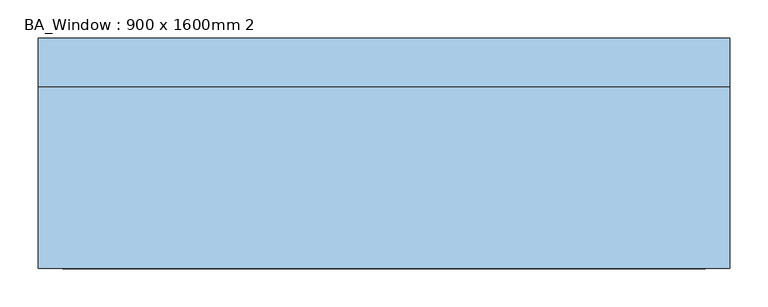
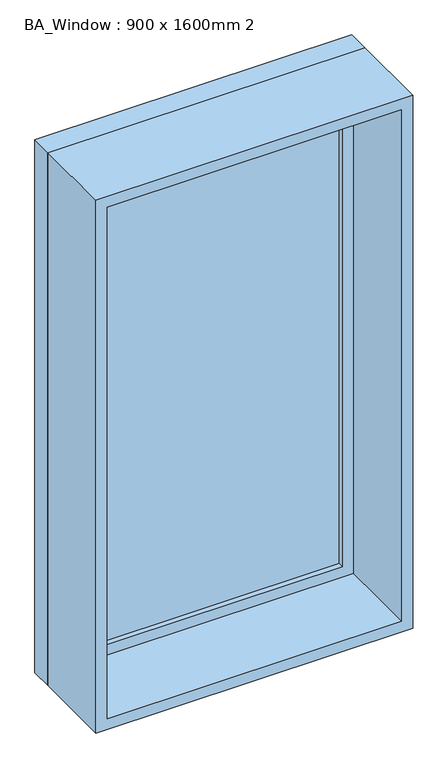
"""IFC4 building model written with IfcOpenShell, lengths in millimetres: window geometry, BA_Window : 900 x 1600mm 2."""

import ifcopenshell
import ifcopenshell.guid

model = None  # the IFC model being written
_history = None  # IfcOwnerHistory: only IFC2X3 demands one
_inside = {}  # id of a spatial element -> (the spatial element, [elements in it])
_under = {}  # id of a project, library or spatial element -> (it, [spatial elements below it])
_declared = {}  # id of a project -> (the project, [libraries it declares])
_typed = {}  # id of a type object -> (the type object, [elements of that type])
_made_of = {}  # id of a material, layer set ... -> (it, [elements and type objects made of it])


def new_model(schema):
    """Start an empty IFC model of exactly this schema.

    Asked for "IFC4X3", IfcOpenShell would pick the latest addendum, in which some entities
    have other attributes; the version numbers below select the first issue.
    IFC2X3 requires an IfcOwnerHistory on every rooted entity: one is made here for all.
    """
    global model, _history
    if schema == "IFC4X3":
        model = ifcopenshell.file(schema_version=(4, 3, 0, 0))
    else:
        model = ifcopenshell.file(schema=schema)
    _inside.clear()
    _under.clear()
    _declared.clear()
    _typed.clear()
    _made_of.clear()
    _history = None
    if model.schema == "IFC2X3":
        org = make("IfcOrganization", Name="unknown")
        user = make(
            "IfcPersonAndOrganization",
            ThePerson=make("IfcPerson", FamilyName="unknown"),
            TheOrganization=org,
        )
        app = make(
            "IfcApplication",
            ApplicationDeveloper=org,
            Version="unknown",
            ApplicationFullName="unknown",
            ApplicationIdentifier="unknown",
        )
        _history = make(
            "IfcOwnerHistory",
            OwningUser=user,
            OwningApplication=app,
            ChangeAction="ADDED",
            CreationDate=0,
        )
    return model


def make(cls, **values):
    """One entity of the class cls with the attributes given. An attribute that is None is left unset."""
    return model.create_entity(
        cls, **{name: value for name, value in values.items() if value is not None}
    )


def rooted(cls, **values):
    """An entity with a GlobalId (a new one), such as an element, a storey or a relation."""
    return make(cls, GlobalId=ifcopenshell.guid.new(), OwnerHistory=_history, **values)


def si_unit(unit_type, name, prefix=None):
    """IfcSIUnit, for example si_unit("LENGTHUNIT", "METRE", prefix="MILLI")."""
    return make("IfcSIUnit", UnitType=unit_type, Prefix=prefix, Name=name)


def assignment(units):
    """IfcUnitAssignment: the units of a project."""
    return None if units is None else make("IfcUnitAssignment", Units=units)


def point(xyz):
    """IfcCartesianPoint."""
    return None if xyz is None else make("IfcCartesianPoint", Coordinates=xyz)


def direction(xyz):
    """IfcDirection."""
    return None if xyz is None else make("IfcDirection", DirectionRatios=xyz)


def frame(location, z_axis=None, x_axis=None):
    """IfcAxis2Placement3D, a coordinate frame: its origin and axes. An axis left out is left unset."""
    return make(
        "IfcAxis2Placement3D",
        Location=point(location),
        Axis=direction(z_axis),
        RefDirection=direction(x_axis),
    )


def origin():
    """The frame at (0, 0, 0) with its axes left unset."""
    return frame((0.0, 0.0, 0.0))


def place(relative_to, where):
    """IfcLocalPlacement: puts the frame where relative to a parent placement (None: the world)."""
    return make(
        "IfcLocalPlacement", PlacementRelTo=relative_to, RelativePlacement=where
    )


def context(
    kind, dimensions, precision=None, world=None, true_north=None, identifier=None
):
    """IfcGeometricRepresentationContext, for example the 3D "Model" context."""
    return make(
        "IfcGeometricRepresentationContext",
        ContextIdentifier=identifier,
        ContextType=kind,
        CoordinateSpaceDimension=dimensions,
        Precision=precision,
        WorldCoordinateSystem=world,
        TrueNorth=true_north,
    )


def project(units=None, contexts=None):
    """IfcProject with its units and contexts."""
    return rooted(
        "IfcProject",
        Name="project",
        RepresentationContexts=contexts,
        UnitsInContext=assignment(units),
    )


def spatial(cls, under=None, at=None, **own):
    """A site, building, storey or space (cls), placed at a placement, below another one or the project."""
    s = rooted(cls, ObjectPlacement=at, **own)
    if under is not None:
        _under.setdefault(under.id(), (under, []))[1].append(s)
    return s


def polyline(points):
    """IfcPolyline through the points."""
    return make("IfcPolyline", Points=[point(p) for p in points])


def outline(outer, holes=None, kind="AREA"):
    """IfcArbitraryClosedProfileDef: a profile drawn as a closed curve; with holes, ...WithVoids."""
    if holes is None:
        return make("IfcArbitraryClosedProfileDef", ProfileType=kind, OuterCurve=outer)
    return make(
        "IfcArbitraryProfileDefWithVoids",
        ProfileType=kind,
        OuterCurve=outer,
        InnerCurves=holes,
    )


def extrude(swept, where, along, depth):
    """IfcExtrudedAreaSolid: the profile swept, set in the frame where, extruded along a direction by depth."""
    return make(
        "IfcExtrudedAreaSolid",
        SweptArea=swept,
        Position=where,
        ExtrudedDirection=direction(along),
        Depth=depth,
    )


def shape(context_of_items, identifier, shape_type, items):
    """IfcShapeRepresentation: the items that make up one representation, for example the "Body"."""
    return make(
        "IfcShapeRepresentation",
        ContextOfItems=context_of_items,
        RepresentationIdentifier=identifier,
        RepresentationType=shape_type,
        Items=items,
    )


def source(mapping_origin, context_of_items, identifier, shape_type, items):
    """IfcRepresentationMap: a shape defined once, which mapped items show again and again."""
    return make(
        "IfcRepresentationMap",
        MappingOrigin=mapping_origin,
        MappedRepresentation=shape(context_of_items, identifier, shape_type, items),
    )


def transform(
    local_origin,
    x_axis=None,
    y_axis=None,
    z_axis=None,
    scale=None,
    scale2=None,
    scale3=None,
    uniform=True,
):
    """IfcCartesianTransformationOperator3D, or its non-uniform kind. x_axis, y_axis, z_axis: its Axis1, 2, 3."""
    if uniform:
        return make(
            "IfcCartesianTransformationOperator3D",
            Axis1=direction(x_axis),
            Axis2=direction(y_axis),
            LocalOrigin=point(local_origin),
            Scale=scale,
            Axis3=direction(z_axis),
        )
    return make(
        "IfcCartesianTransformationOperator3DnonUniform",
        Axis1=direction(x_axis),
        Axis2=direction(y_axis),
        LocalOrigin=point(local_origin),
        Scale=scale,
        Axis3=direction(z_axis),
        Scale2=scale2,
        Scale3=scale3,
    )


def mapped(mapping_source, mapping_target):
    """IfcMappedItem: shows the shape of a source again, moved by a transform."""
    return make(
        "IfcMappedItem", MappingSource=mapping_source, MappingTarget=mapping_target
    )


def made_of(thing, what):
    """Note that an element or type object is made of a material, layer set ...; save() writes the relation."""
    if what is not None:
        _made_of.setdefault(what.id(), (what, []))[1].append(thing)
    return thing


def element(
    cls,
    number,
    at=None,
    inside=None,
    cuts=None,
    type_object=None,
    material=None,
    context=None,
    identifier="Body",
    shape_type=None,
    held_by="IfcProductDefinitionShape",
    body=None,
    shapes=None,
    **own,
):
    """One element of the class cls, such as IfcWall. Its Tag is "e" and its number.

    at: its placement. inside: the storey or other place that contains it. cuts: it is an
    opening in that element (IfcRelVoidsElement). A single representation is given by context,
    identifier, shape_type and body (its items); several are given by shapes. held_by: the class
    of the entity that holds the representations. save() writes the other relations.
    """
    e = rooted(cls, Tag="e%d" % number, ObjectPlacement=at, **own)
    if body is not None:
        shapes = [shape(context, identifier, shape_type, body)]
    if shapes is not None:
        e.Representation = make(held_by, Representations=shapes)
    if inside is not None:
        _inside.setdefault(inside.id(), (inside, []))[1].append(e)
    if cuts is not None:
        rooted(
            "IfcRelVoidsElement", RelatingBuildingElement=cuts, RelatedOpeningElement=e
        )
    if type_object is not None:
        _typed.setdefault(type_object.id(), (type_object, []))[1].append(e)
    return made_of(e, material)


def aggregate(whole, parts):
    """IfcRelAggregates: a whole, such as a stair, and the parts it consists of."""
    return rooted("IfcRelAggregates", RelatingObject=whole, RelatedObjects=parts)


def save(model, path):
    """Write the relations noted so far, then the file.

    IfcRelAggregates (storeys below a building ...), IfcRelContainedInSpatialStructure (elements
    in a storey), IfcRelDefinesByType, IfcRelAssociatesMaterial and IfcRelDeclares: one each for
    every whole, place, type object, material and project.
    """
    for whole, parts in _under.values():
        aggregate(whole, parts)
    for where, things in _inside.values():
        rooted(
            "IfcRelContainedInSpatialStructure",
            RelatedElements=things,
            RelatingStructure=where,
        )
    for kind, things in _typed.values():
        rooted("IfcRelDefinesByType", RelatedObjects=things, RelatingType=kind)
    for what, things in _made_of.values():
        rooted("IfcRelAssociatesMaterial", RelatedObjects=things, RelatingMaterial=what)
    for by, libraries in _declared.values():
        rooted("IfcRelDeclares", RelatingContext=by, RelatedDefinitions=libraries)
    model.write(path)


def ba_window_900_x_1600mm_2_0de2e490(model_context):
    return source(origin(), model_context, "Body", "SweptSolid", [
        extrude(outline(polyline([(-387.0, 128.0), (387.0, 128.0), (387.0, 116.0), (-387.0, 116.0), (-387.0, 128.0)])), frame((0.0, 0.0, 978.0), z_axis=(0.0, 0.0, 1.0), x_axis=(1.0, 0.0, 0.0)), (0.0, 0.0, 1.0), 1474.0),
        extrude(outline(polyline([(2496.0, -431.0), (934.0, -431.0), (934.0, 431.0), (2496.0, 431.0), (2496.0, -431.0)]), holes=[polyline([(2452.0, -387.0), (2452.0, 387.0), (978.0, 387.0), (978.0, -387.0), (2452.0, -387.0)])]), frame((0.0, 100.0, 0.0), z_axis=(0.0, 1.0, 0.0), x_axis=(0.0, 0.0, 1.0)), (0.0, 0.0, 1.0), 44.0),
        extrude(outline(polyline([(2515.0, -450.0), (915.0, -450.0), (915.0, 450.0), (2515.0, 450.0), (2515.0, -450.0)]), holes=[polyline([(2496.0, -431.0), (2496.0, 431.0), (934.0, 431.0), (934.0, -431.0), (2496.0, -431.0)])]), frame((0.0, 100.0, 0.0), z_axis=(0.0, 1.0, 0.0), x_axis=(0.0, 0.0, 1.0)), (0.0, 0.0, 1.0), 63.0),
        extrude(outline(polyline([(2515.0, -450.0), (915.0, -450.0), (915.0, 450.0), (2515.0, 450.0), (2515.0, -450.0)]), holes=[polyline([(2483.0, -418.0), (2483.0, 418.0), (947.0, 418.0), (947.0, -418.0), (2483.0, -418.0)])]), frame((0.0, -137.0, 0.0), z_axis=(0.0, 1.0, 0.0), x_axis=(0.0, 0.0, 1.0)), (0.0, 0.0, 1.0), 237.0),
    ])


if __name__ == "__main__":
    model = new_model("IFC4")
    model_context = context("Model", 3, world=origin())
    ifc_project = project(units=[si_unit("LENGTHUNIT", "METRE", prefix="MILLI")], contexts=[model_context])
    site = spatial("IfcSite", under=ifc_project)
    building = spatial("IfcBuilding", under=site)
    placement = place(None, origin())
    ba_window_900_x_1600mm_2_shape = ba_window_900_x_1600mm_2_0de2e490(model_context)
    element("IfcWindow", 1, ObjectType="BA_Window : 900 x 1600mm 2", at=placement, inside=building, context=model_context, shape_type="MappedRepresentation", body=[
        mapped(ba_window_900_x_1600mm_2_shape, transform((0.0, 0.0, 0.0), x_axis=(1.0, 0.0, 0.0), y_axis=(0.0, 1.0, 0.0), z_axis=(0.0, 0.0, 1.0))),
    ])
    save(model, "model.ifc")

# Revit data of these elements
# Type "BA_Window : 900 x 1600mm 2"
#   Type Mark = "40"
#   Construction Type Id = "GSP4R"
#   Analytic Construction = "1/8 in Pilkington single glazing"
#   Visual Light Transmittance = 0.9
#   Thermal Resistance (R) = 0.271106 (m²·K)/W
#   Solar Heat Gain Coefficient = 0.78
#   Heat Transfer Coefficient (U) = 3.6886 W/(m²·K)
#   Height = 1600 mm
#   Default Sill Height = 915 mm
#   Width = 900 mm
#   Window Inset = 19 mm
#   Define Thermal Properties by = 1
#   Frame Exterior Material = Default
#   Frame Interior Material = Default
#   Glass Pane Material = Glass
#   Sash = Default
#   Wall Closure = (empty or 0)
# Element 1 (IfcWindow, "BA_Window : 900 x 1600mm 2")
#   Materials on its faces: "Default", "Glass"
# Materials
#   "Default": class "Generic", colour RGB 255 255 255, transparency 0, Cost = 0
#   "Glass": class "Glass", colour RGB 0 128 192, transparency 0.9, Description = "Soda Lime Glass", Cost = 0
